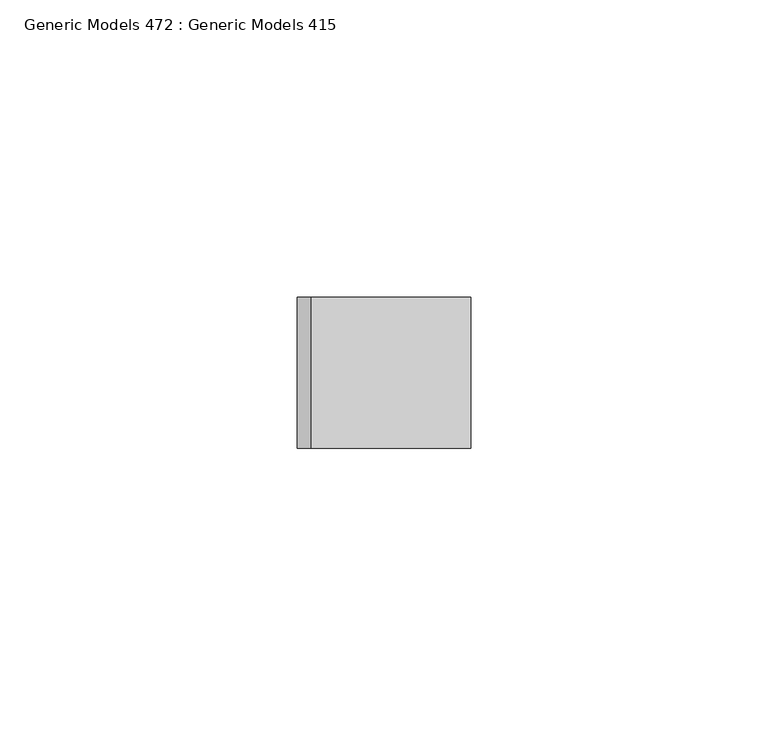
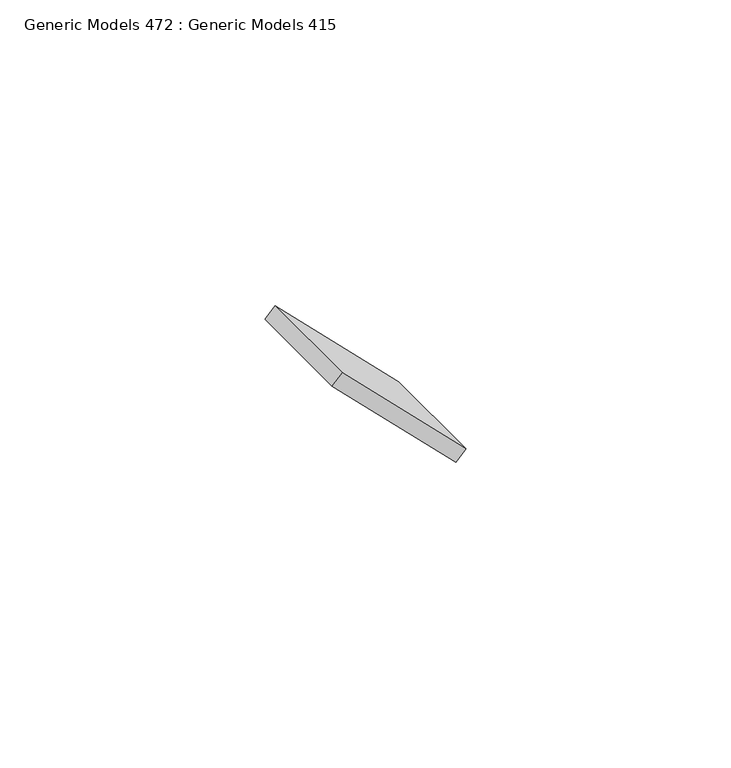
"""IFC4 building model written with IfcOpenShell, lengths in millimetres: proxy geometry, Generic Models 472 : Generic Models 415."""

from ifc_helpers import new_model, si_unit, frame, origin, place, context, project, spatial, polyline, outline, extrude, source, transform, mapped, element, save


def generic_models_472_generic_models_415_1bea41d2(model_context):
    return source(origin(), model_context, "Body", "SweptSolid", [
        extrude(outline(polyline([(0.0, -38.1), (0.0, 0.0), (25.4, 0.0), (25.4, -38.1), (0.0, -38.1)])), frame((-6869.8996186, -4475.9863946, 128099.0002957), z_axis=(0.7071067811864907, 0.0, 0.7071067811866044), x_axis=(0.0, -1.0, 0.0)), (0.0, 0.0, 1.0), 3.175),
    ])


if __name__ == "__main__":
    model = new_model("IFC4")
    model_context = context("Model", 3, world=origin())
    ifc_project = project(units=[si_unit("LENGTHUNIT", "METRE", prefix="MILLI")], contexts=[model_context])
    site = spatial("IfcSite", under=ifc_project)
    building = spatial("IfcBuilding", under=site)
    placement = place(None, origin())
    generic_models_472_generic_models_415_shape = generic_models_472_generic_models_415_1bea41d2(model_context)
    element("IfcBuildingElementProxy", 1, Name="Generic Models 472 : Generic Models 415", ObjectType="Generic Models 472 : Generic Models 415", at=placement, inside=building, context=model_context, shape_type="MappedRepresentation", body=[
        mapped(generic_models_472_generic_models_415_shape, transform((0.0, 0.0, 0.0), x_axis=(1.0, 0.0, 0.0), y_axis=(0.0, 1.0, 0.0), z_axis=(0.0, 0.0, 1.0))),
    ])
    save(model, "model.ifc")

# Revit data of these elements
# Element 1 (IfcBuildingElementProxy, "Generic Models 472 : Generic Models 415")
#   Materials on its faces: "_WELDED STEEL TABS FOR LOUVER ATTACHMENT"
# Materials
#   "_WELDED STEEL TABS FOR LOUVER ATTACHMENT": class "Metal", colour RGB 199 199 199, transparency 0, Description = "Structural steel 50ksi", Cost = 0
